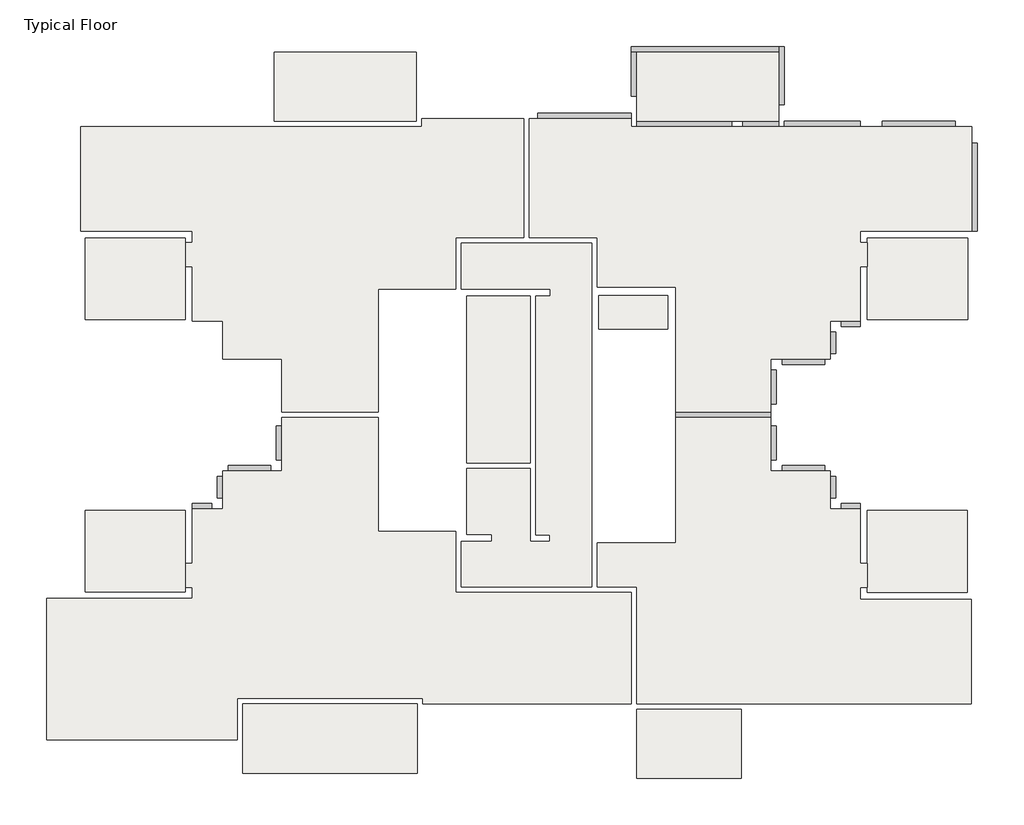
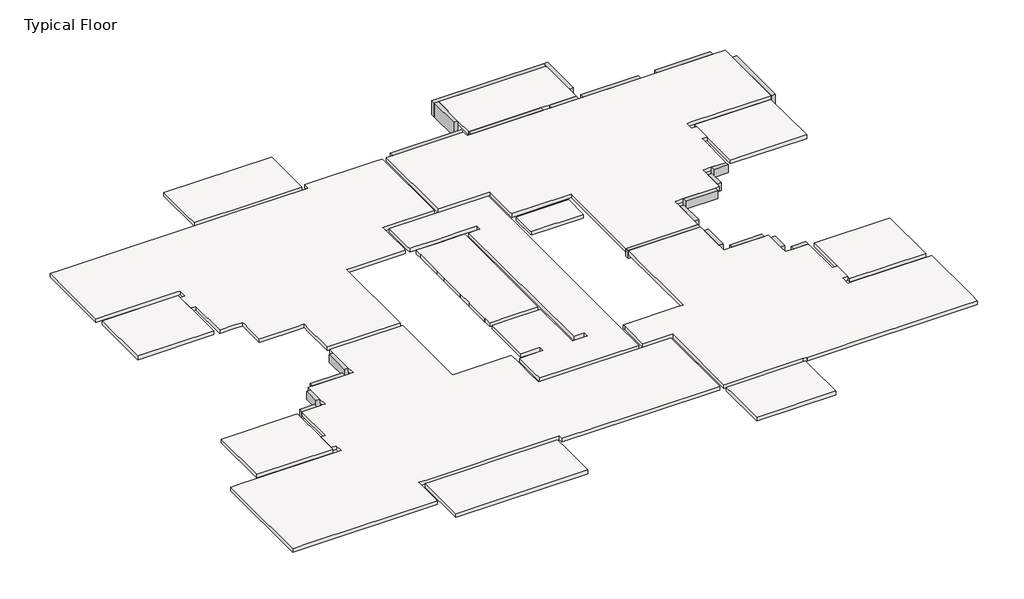
# One storey: 22 beams, 15 slabs.
"""IFC4 building model written with IfcOpenShell, lengths in millimetres."""

import ifcopenshell
import ifcopenshell.guid

model = None  # the IFC model being written
_history = None  # IfcOwnerHistory: only IFC2X3 demands one
_inside = {}  # id of a spatial element -> (the spatial element, [elements in it])
_under = {}  # id of a project, library or spatial element -> (it, [spatial elements below it])
_declared = {}  # id of a project -> (the project, [libraries it declares])
_typed = {}  # id of a type object -> (the type object, [elements of that type])
_made_of = {}  # id of a material, layer set ... -> (it, [elements and type objects made of it])


def new_model(schema):
    """Start an empty IFC model of exactly this schema.

    Asked for "IFC4X3", IfcOpenShell would pick the latest addendum, in which some entities
    have other attributes; the version numbers below select the first issue.
    IFC2X3 requires an IfcOwnerHistory on every rooted entity: one is made here for all.
    """
    global model, _history
    if schema == "IFC4X3":
        model = ifcopenshell.file(schema_version=(4, 3, 0, 0))
    else:
        model = ifcopenshell.file(schema=schema)
    _inside.clear()
    _under.clear()
    _declared.clear()
    _typed.clear()
    _made_of.clear()
    _history = None
    if model.schema == "IFC2X3":
        org = make("IfcOrganization", Name="unknown")
        user = make(
            "IfcPersonAndOrganization",
            ThePerson=make("IfcPerson", FamilyName="unknown"),
            TheOrganization=org,
        )
        app = make(
            "IfcApplication",
            ApplicationDeveloper=org,
            Version="unknown",
            ApplicationFullName="unknown",
            ApplicationIdentifier="unknown",
        )
        _history = make(
            "IfcOwnerHistory",
            OwningUser=user,
            OwningApplication=app,
            ChangeAction="ADDED",
            CreationDate=0,
        )
    return model


def make(cls, **values):
    """One entity of the class cls with the attributes given. An attribute that is None is left unset."""
    return model.create_entity(
        cls, **{name: value for name, value in values.items() if value is not None}
    )


def rooted(cls, **values):
    """An entity with a GlobalId (a new one), such as an element, a storey or a relation."""
    return make(cls, GlobalId=ifcopenshell.guid.new(), OwnerHistory=_history, **values)


def si_unit(unit_type, name, prefix=None):
    """IfcSIUnit, for example si_unit("LENGTHUNIT", "METRE", prefix="MILLI")."""
    return make("IfcSIUnit", UnitType=unit_type, Prefix=prefix, Name=name)


def assignment(units):
    """IfcUnitAssignment: the units of a project."""
    return None if units is None else make("IfcUnitAssignment", Units=units)


def point(xyz):
    """IfcCartesianPoint."""
    return None if xyz is None else make("IfcCartesianPoint", Coordinates=xyz)


def direction(xyz):
    """IfcDirection."""
    return None if xyz is None else make("IfcDirection", DirectionRatios=xyz)


def frame(location, z_axis=None, x_axis=None):
    """IfcAxis2Placement3D, a coordinate frame: its origin and axes. An axis left out is left unset."""
    return make(
        "IfcAxis2Placement3D",
        Location=point(location),
        Axis=direction(z_axis),
        RefDirection=direction(x_axis),
    )


def origin():
    """The frame at (0, 0, 0) with its axes left unset."""
    return frame((0.0, 0.0, 0.0))


def place(relative_to, where):
    """IfcLocalPlacement: puts the frame where relative to a parent placement (None: the world)."""
    return make(
        "IfcLocalPlacement", PlacementRelTo=relative_to, RelativePlacement=where
    )


def context(
    kind, dimensions, precision=None, world=None, true_north=None, identifier=None
):
    """IfcGeometricRepresentationContext, for example the 3D "Model" context."""
    return make(
        "IfcGeometricRepresentationContext",
        ContextIdentifier=identifier,
        ContextType=kind,
        CoordinateSpaceDimension=dimensions,
        Precision=precision,
        WorldCoordinateSystem=world,
        TrueNorth=true_north,
    )


def project(units=None, contexts=None):
    """IfcProject with its units and contexts."""
    return rooted(
        "IfcProject",
        Name="project",
        RepresentationContexts=contexts,
        UnitsInContext=assignment(units),
    )


def spatial(cls, under=None, at=None, **own):
    """A site, building, storey or space (cls), placed at a placement, below another one or the project."""
    s = rooted(cls, ObjectPlacement=at, **own)
    if under is not None:
        _under.setdefault(under.id(), (under, []))[1].append(s)
    return s


def polyline(points):
    """IfcPolyline through the points."""
    return make("IfcPolyline", Points=[point(p) for p in points])


def outline(outer, holes=None, kind="AREA"):
    """IfcArbitraryClosedProfileDef: a profile drawn as a closed curve; with holes, ...WithVoids."""
    if holes is None:
        return make("IfcArbitraryClosedProfileDef", ProfileType=kind, OuterCurve=outer)
    return make(
        "IfcArbitraryProfileDefWithVoids",
        ProfileType=kind,
        OuterCurve=outer,
        InnerCurves=holes,
    )


def extrude(swept, where, along, depth):
    """IfcExtrudedAreaSolid: the profile swept, set in the frame where, extruded along a direction by depth."""
    return make(
        "IfcExtrudedAreaSolid",
        SweptArea=swept,
        Position=where,
        ExtrudedDirection=direction(along),
        Depth=depth,
    )


def faces_of(points, faces, orient=None, outer=None):
    """IfcFace entities. A face is a list of loops; a loop is a list of indices into points, from 0.

    orient and outer hold one flag for each loop. By default every Orientation is true, the
    first loop of a face is its IfcFaceOuterBound and the others are IfcFaceBound.
    """
    made = []
    for i, loops in enumerate(faces):
        bounds = []
        for j, loop in enumerate(loops):
            is_outer = j == 0 if outer is None else outer[i][j]
            bounds.append(
                make(
                    "IfcFaceOuterBound" if is_outer else "IfcFaceBound",
                    Bound=make("IfcPolyLoop", Polygon=[points[k] for k in loop]),
                    Orientation=True if orient is None else orient[i][j],
                )
            )
        made.append(make("IfcFace", Bounds=bounds))
    return made


def faceted_brep(points, faces, orient=None, outer=None, voids=None):
    """IfcFacetedBrep: a solid bounded by flat faces; with voids (closed shells), ...WithVoids."""
    shared = [point(p) for p in points]
    hull = make("IfcClosedShell", CfsFaces=faces_of(shared, faces, orient, outer))
    if voids is None:
        return make("IfcFacetedBrep", Outer=hull)
    return make(
        "IfcFacetedBrepWithVoids",
        Outer=hull,
        Voids=[
            make(cls, CfsFaces=faces_of(shared, fs, o, b)) for cls, fs, o, b in voids
        ],
    )


def shape(context_of_items, identifier, shape_type, items):
    """IfcShapeRepresentation: the items that make up one representation, for example the "Body"."""
    return make(
        "IfcShapeRepresentation",
        ContextOfItems=context_of_items,
        RepresentationIdentifier=identifier,
        RepresentationType=shape_type,
        Items=items,
    )


def made_of(thing, what):
    """Note that an element or type object is made of a material, layer set ...; save() writes the relation."""
    if what is not None:
        _made_of.setdefault(what.id(), (what, []))[1].append(thing)
    return thing


def element(
    cls,
    number,
    at=None,
    inside=None,
    cuts=None,
    type_object=None,
    material=None,
    context=None,
    identifier="Body",
    shape_type=None,
    held_by="IfcProductDefinitionShape",
    body=None,
    shapes=None,
    **own,
):
    """One element of the class cls, such as IfcWall. Its Tag is "e" and its number.

    at: its placement. inside: the storey or other place that contains it. cuts: it is an
    opening in that element (IfcRelVoidsElement). A single representation is given by context,
    identifier, shape_type and body (its items); several are given by shapes. held_by: the class
    of the entity that holds the representations. save() writes the other relations.
    """
    e = rooted(cls, Tag="e%d" % number, ObjectPlacement=at, **own)
    if body is not None:
        shapes = [shape(context, identifier, shape_type, body)]
    if shapes is not None:
        e.Representation = make(held_by, Representations=shapes)
    if inside is not None:
        _inside.setdefault(inside.id(), (inside, []))[1].append(e)
    if cuts is not None:
        rooted(
            "IfcRelVoidsElement", RelatingBuildingElement=cuts, RelatedOpeningElement=e
        )
    if type_object is not None:
        _typed.setdefault(type_object.id(), (type_object, []))[1].append(e)
    return made_of(e, material)


def aggregate(whole, parts):
    """IfcRelAggregates: a whole, such as a stair, and the parts it consists of."""
    return rooted("IfcRelAggregates", RelatingObject=whole, RelatedObjects=parts)


def save(model, path):
    """Write the relations noted so far, then the file.

    IfcRelAggregates (storeys below a building ...), IfcRelContainedInSpatialStructure (elements
    in a storey), IfcRelDefinesByType, IfcRelAssociatesMaterial and IfcRelDeclares: one each for
    every whole, place, type object, material and project.
    """
    for whole, parts in _under.values():
        aggregate(whole, parts)
    for where, things in _inside.values():
        rooted(
            "IfcRelContainedInSpatialStructure",
            RelatedElements=things,
            RelatingStructure=where,
        )
    for kind, things in _typed.values():
        rooted("IfcRelDefinesByType", RelatedObjects=things, RelatingType=kind)
    for what, things in _made_of.values():
        rooted("IfcRelAssociatesMaterial", RelatedObjects=things, RelatingMaterial=what)
    for by, libraries in _declared.values():
        rooted("IfcRelDeclares", RelatingContext=by, RelatedDefinitions=libraries)
    model.write(path)


model = new_model("IFC4")

# Units and contexts
model_context = context("Model", 3, world=origin())
ifc_project = project(units=[si_unit("LENGTHUNIT", "METRE", prefix="MILLI")], contexts=[model_context])

# Site, building, storey
site = spatial("IfcSite", under=ifc_project)
building = spatial("IfcBuilding", under=site)
storey = spatial("IfcBuildingStorey", under=building, Name="Typical Floor", Elevation=3200.0)

# Beams
placement = place(None, origin())
element("IfcBeam", 1, ObjectType="Concrete Rectengular Beam : 20/40", at=placement, inside=storey, context=model_context, shape_type="Brep", body=[
    faceted_brep([(12187.8813243, 1505.2784849, 3200.0), (12187.8813243, 1705.2784849, 3200.0), (11489.3591568, 1705.2784849, 3200.0), (11489.3591568, 1505.2784849, 3200.0), (12187.8813243, 1705.2784849, 3020.0), (12187.8813243, 1705.2784849, 2800.0), (11489.3591568, 1705.2784849, 2800.0), (12187.8813243, 1505.2784849, 2800.0), (11489.3591568, 1505.2784849, 2800.0)], [[[0, 1, 2, 3]], [[1, 4, 5, 6, 2]], [[5, 7, 8, 6]], [[7, 0, 3, 8]], [[1, 0, 7, 5, 4]], [[3, 2, 6, 8]]]),
])
element("IfcBeam", 2, ObjectType="Concrete Rectengular Beam : 20/40", at=placement, inside=storey, context=model_context, shape_type="SweptSolid", body=[
    extrude(outline(polyline([(11289.3591568, 525.2784849), (11089.3591568, 525.2784849), (11089.3591568, 1305.2784849), (11289.3591568, 1305.2784849), (11289.3591568, 525.2784849)])), frame((0.0, 0.0, 2800.0), z_axis=(0.0, 0.0, 1.0), x_axis=(1.0, 0.0, 0.0)), (0.0, 0.0, 1.0), 400.0),
])
element("IfcBeam", 3, ObjectType="Concrete Rectengular Beam : 20/40", at=placement, inside=storey, context=model_context, shape_type="SweptSolid", body=[
    extrude(outline(polyline([(9356.052096, 125.2784849), (9356.052096, 325.2784849), (10889.3591568, 325.2784849), (10889.3591568, 125.2784849), (9356.052096, 125.2784849)])), frame((0.0, 0.0, 2800.0), z_axis=(0.0, 0.0, 1.0), x_axis=(1.0, 0.0, 0.0)), (0.0, 0.0, 1.0), 400.0),
])
element("IfcBeam", 4, ObjectType="Concrete Rectengular Beam : 20/40", at=placement, inside=storey, context=model_context, shape_type="Brep", body=[
    faceted_brep([(8956.052096, -1293.9530422, 3200.0), (9156.052096, -1293.9530422, 3200.0), (9156.052096, -74.7215151, 3200.0), (8956.052096, -74.7215151, 3200.0), (9156.052096, -1293.9530422, 2800.0), (9156.052096, -74.7215151, 2800.0), (8956.052096, -1293.9530422, 2800.0), (8956.052096, -74.7215151, 2800.0), (8956.052096, -1293.9530422, 3020.0)], [[[0, 1, 2, 3]], [[1, 4, 5, 2]], [[4, 6, 7, 5]], [[6, 8, 0, 3, 7]], [[1, 0, 8, 6, 4]], [[3, 2, 5, 7]]]),
])
element("IfcBeam", 5, ObjectType="Concrete Rectengular Beam : 20/40", at=placement, inside=storey, context=model_context, shape_type="Brep", body=[
    faceted_brep([(8956.052096, -1793.9530422, 3200.0), (8956.052096, -1593.9530422, 3200.0), (5525.8815794, -1593.9530422, 3200.0), (5525.8815794, -1793.9530422, 3200.0), (8956.052096, -1793.9530422, 2800.0), (8956.052096, -1793.9530422, 3020.0), (5525.8815794, -1793.9530422, 3020.0), (5525.8815794, -1793.9530422, 2800.0), (8956.052096, -1593.9530422, 2800.0), (5525.8815794, -1593.9530422, 2800.0), (8956.052096, -1593.9530422, 3020.0), (5525.8815794, -1593.9530422, 3020.0)], [[[0, 1, 2, 3]], [[4, 5, 0, 3, 6, 7]], [[8, 4, 7, 9]], [[1, 10, 8, 9, 11, 2]], [[1, 0, 5, 4, 8, 10]], [[3, 2, 11, 9, 7, 6]]]),
])
element("IfcBeam", 6, ObjectType="Concrete Rectengular Beam : 20/40", at=placement, inside=storey, context=model_context, shape_type="Brep", body=[
    faceted_brep([(-11929.8186713, -4893.1845693, 3200.0), (-11929.8186713, -5093.1845693, 3200.0), (-11231.2965038, -5093.1845693, 3200.0), (-11231.2965038, -4893.1845693, 3200.0), (-11929.8186713, -5093.1845693, 3020.0), (-11929.8186713, -5093.1845693, 2800.0), (-11231.2965038, -5093.1845693, 2800.0), (-11929.8186713, -4893.1845693, 2800.0), (-11231.2965038, -4893.1845693, 2800.0)], [[[0, 1, 2, 3]], [[1, 4, 5, 6, 2]], [[5, 7, 8, 6]], [[7, 0, 3, 8]], [[1, 0, 7, 5, 4]], [[3, 2, 6, 8]]]),
])
element("IfcBeam", 7, ObjectType="Concrete Rectengular Beam : 20/40", at=placement, inside=storey, context=model_context, shape_type="SweptSolid", body=[
    extrude(outline(polyline([(-11031.2965038, -3913.1845693), (-10831.2965038, -3913.1845693), (-10831.2965038, -4693.1845693), (-11031.2965038, -4693.1845693), (-11031.2965038, -3913.1845693)])), frame((0.0, 0.0, 2800.0), z_axis=(0.0, 0.0, 1.0), x_axis=(1.0, 0.0, 0.0)), (0.0, 0.0, 1.0), 400.0),
])
element("IfcBeam", 8, ObjectType="Concrete Rectengular Beam : 20/40", at=placement, inside=storey, context=model_context, shape_type="SweptSolid", body=[
    extrude(outline(polyline([(-9097.9894431, -3513.1845693), (-9097.9894431, -3713.1845693), (-10631.2965038, -3713.1845693), (-10631.2965038, -3513.1845693), (-9097.9894431, -3513.1845693)])), frame((0.0, 0.0, 2800.0), z_axis=(0.0, 0.0, 1.0), x_axis=(1.0, 0.0, 0.0)), (0.0, 0.0, 1.0), 400.0),
])
element("IfcBeam", 9, ObjectType="Concrete Rectengular Beam : 20/40", at=placement, inside=storey, context=model_context, shape_type="Brep", body=[
    faceted_brep([(-8697.9894431, -2093.9530422, 3200.0), (-8897.9894431, -2093.9530422, 3200.0), (-8897.9894431, -3313.1845693, 3200.0), (-8697.9894431, -3313.1845693, 3200.0), (-8897.9894431, -2093.9530422, 2800.0), (-8897.9894431, -3313.1845693, 2800.0), (-8697.9894431, -2093.9530422, 2800.0), (-8697.9894431, -3313.1845693, 2800.0), (-8697.9894431, -2093.9530422, 3020.0)], [[[0, 1, 2, 3]], [[1, 4, 5, 2]], [[4, 6, 7, 5]], [[6, 8, 0, 3, 7]], [[1, 0, 8, 6, 4]], [[3, 2, 5, 7]]]),
])
element("IfcBeam", 10, ObjectType="Concrete Rectengular Beam : 20/40", at=placement, inside=storey, context=model_context, shape_type="Brep", body=[
    faceted_brep([(12187.8813243, -5093.1845693, 3200.0), (12187.8813243, -4893.1845693, 3200.0), (11489.3591568, -4893.1845693, 3200.0), (11489.3591568, -5093.1845693, 3200.0), (12187.8813243, -5093.1845693, 2800.0), (12187.8813243, -5093.1845693, 3020.0), (11489.3591568, -5093.1845693, 2800.0), (12187.8813243, -4893.1845693, 2800.0), (11489.3591568, -4893.1845693, 2800.0)], [[[0, 1, 2, 3]], [[4, 5, 0, 3, 6]], [[7, 4, 6, 8]], [[1, 7, 8, 2]], [[1, 0, 5, 4, 7]], [[3, 2, 8, 6]]]),
])
element("IfcBeam", 11, ObjectType="Concrete Rectengular Beam : 20/40", at=placement, inside=storey, context=model_context, shape_type="SweptSolid", body=[
    extrude(outline(polyline([(11289.3591568, -4693.1845693), (11089.3591568, -4693.1845693), (11089.3591568, -3913.1845693), (11289.3591568, -3913.1845693), (11289.3591568, -4693.1845693)])), frame((0.0, 0.0, 2800.0), z_axis=(0.0, 0.0, 1.0), x_axis=(1.0, 0.0, 0.0)), (0.0, 0.0, 1.0), 400.0),
])
element("IfcBeam", 12, ObjectType="Concrete Rectengular Beam : 20/40", at=placement, inside=storey, context=model_context, shape_type="SweptSolid", body=[
    extrude(outline(polyline([(10889.3591568, -3513.1845693), (10889.3591568, -3713.1845693), (9356.052096, -3713.1845693), (9356.052096, -3513.1845693), (10889.3591568, -3513.1845693)])), frame((0.0, 0.0, 2800.0), z_axis=(0.0, 0.0, 1.0), x_axis=(1.0, 0.0, 0.0)), (0.0, 0.0, 1.0), 400.0),
])
element("IfcBeam", 13, ObjectType="Concrete Rectengular Beam : 20/40", at=placement, inside=storey, context=model_context, shape_type="Brep", body=[
    faceted_brep([(9156.052096, -2093.9530422, 3200.0), (8956.052096, -2093.9530422, 3200.0), (8956.052096, -3313.1845693, 3200.0), (9156.052096, -3313.1845693, 3200.0), (9156.052096, -2093.9530422, 2800.0), (9156.052096, -3313.1845693, 2800.0), (8956.052096, -2093.9530422, 2800.0), (8956.052096, -3313.1845693, 2800.0), (8956.052096, -2093.9530422, 3020.0)], [[[0, 1, 2, 3]], [[4, 0, 3, 5]], [[6, 4, 5, 7]], [[1, 8, 6, 7, 2]], [[1, 0, 4, 6, 8]], [[3, 2, 7, 5]]]),
])
element("IfcBeam", 14, ObjectType="Concrete Rectengular Beam : 20/50", at=placement, inside=storey, context=model_context, shape_type="Brep", body=[
    faceted_brep([(4107.8539459, 8914.1448811, 3200.0), (4107.8539459, 8714.1448811, 3200.0), (7543.9303787, 8714.1448811, 3200.0), (7543.9303787, 8914.1448811, 3200.0), (4107.8539459, 8914.1448811, 2700.0), (4107.8539459, 8914.1448811, 3020.0), (7543.9303787, 8914.1448811, 2700.0), (4107.8539459, 8714.1448811, 2700.0), (7543.9303787, 8714.1448811, 2700.0), (4107.8539459, 8714.1448811, 3020.0), (7543.9303787, 8714.1448811, 3020.0)], [[[0, 1, 2, 3]], [[4, 5, 0, 3, 6]], [[7, 4, 6, 8]], [[2, 1, 9, 7, 8, 10]], [[1, 0, 5, 4, 7, 9]], [[3, 2, 10, 8, 6]]]),
])
element("IfcBeam", 15, ObjectType="Concrete Rectengular Beam : 20/50", at=placement, inside=storey, context=model_context, shape_type="Brep", body=[
    faceted_brep([(7943.9303787, 8914.1448811, 3200.0), (7943.9303787, 8714.1448811, 3200.0), (9233.1802646, 8714.1448811, 3200.0), (9233.1802646, 8914.1448811, 3200.0), (7943.9303787, 8914.1448811, 2700.0), (9233.1802646, 8914.1448811, 3020.0), (9233.1802646, 8914.1448811, 2700.0), (7943.9303787, 8714.1448811, 2700.0), (9233.1802646, 8714.1448811, 2700.0), (7943.9303787, 8714.1448811, 3020.0), (9233.1802646, 8714.1448811, 3020.0)], [[[0, 1, 2, 3]], [[4, 0, 3, 5, 6]], [[7, 4, 6, 8]], [[2, 1, 9, 7, 8, 10]], [[1, 0, 4, 7, 9]], [[3, 2, 10, 8, 6, 5]]]),
])
element("IfcBeam", 16, ObjectType="Concrete Rectengular Beam : 20/50", at=placement, inside=storey, context=model_context, shape_type="Brep", body=[
    faceted_brep([(9433.1802646, 8914.1448811, 3200.0), (9433.1802646, 8714.1448811, 3200.0), (12172.2581695, 8714.1448811, 3200.0), (12172.2581695, 8914.1448811, 3200.0), (9433.1802646, 8914.1448811, 2700.0), (12172.2581695, 8914.1448811, 2700.0), (9433.1802646, 8714.1448811, 2700.0), (12172.2581695, 8714.1448811, 2700.0), (9433.1802646, 8714.1448811, 3020.0), (12172.2581695, 8714.1448811, 3020.0)], [[[0, 1, 2, 3]], [[4, 0, 3, 5]], [[6, 4, 5, 7]], [[2, 1, 8, 6, 7, 9]], [[1, 0, 4, 6, 8]], [[3, 2, 9, 7, 5]]]),
])
element("IfcBeam", 17, ObjectType="Concrete Rectengular Beam : 20/50", at=placement, inside=storey, context=model_context, shape_type="Brep", body=[
    faceted_brep([(12972.2581695, 8914.1448811, 3200.0), (12972.2581695, 8714.1448811, 3200.0), (15617.6251666, 8714.1448811, 3200.0), (15617.6251666, 8914.1448811, 3200.0), (12972.2581695, 8914.1448811, 2700.0), (15617.6251666, 8914.1448811, 2700.0), (12972.2581695, 8714.1448811, 2700.0), (15617.6251666, 8714.1448811, 2700.0), (12972.2581695, 8714.1448811, 3020.0), (15617.6251666, 8714.1448811, 3020.0)], [[[0, 1, 2, 3]], [[4, 0, 3, 5]], [[6, 4, 5, 7]], [[2, 1, 8, 6, 7, 9]], [[1, 0, 4, 6, 8]], [[3, 2, 9, 7, 5]]]),
])
element("IfcBeam", 18, ObjectType="Concrete Rectengular Beam : 20/50", at=placement, inside=storey, context=model_context, shape_type="Brep", body=[
    faceted_brep([(16410.4478267, 8125.9123109, 3200.0), (16210.4478267, 8125.9123109, 3200.0), (16210.4478267, 4939.6791417, 3200.0), (16410.4478267, 4939.6791417, 3200.0), (16410.4478267, 8125.9123109, 2700.0), (16410.4478267, 4939.6791417, 2700.0), (16210.4478267, 8125.9123109, 2700.0), (16210.4478267, 4939.6791417, 2700.0), (16210.4478267, 4939.6791417, 3020.0)], [[[0, 1, 2, 3]], [[4, 0, 3, 5]], [[6, 4, 5, 7]], [[1, 6, 7, 8, 2]], [[1, 0, 4, 6]], [[3, 2, 8, 7, 5]]]),
])
element("IfcBeam", 19, ObjectType="Concrete Rectengular Beam : 20/50", at=placement, inside=storey, context=model_context, shape_type="Brep", body=[
    faceted_brep([(3907.8539459, 9014.1448811, 3200.0), (3907.8539459, 9214.1448811, 3200.0), (529.0313265, 9214.1448811, 3200.0), (529.0313265, 9014.1448811, 3200.0), (3907.8539459, 9214.1448811, 2700.0), (529.0313265, 9214.1448811, 2700.0), (3907.8539459, 9014.1448811, 2700.0), (529.0313265, 9014.1448811, 2700.0), (3907.8539459, 9014.1448811, 3020.0)], [[[0, 1, 2, 3]], [[1, 4, 5, 2]], [[4, 6, 7, 5]], [[6, 8, 0, 3, 7]], [[1, 0, 8, 6, 4]], [[3, 2, 5, 7]]]),
])
element("IfcBeam", 20, ObjectType="Concrete Rectengular Beam : 20/70", at=placement, inside=storey, context=model_context, shape_type="Brep", body=[
    faceted_brep([(9433.1802646, 11614.1448811, 3200.0), (9233.1802646, 11614.1448811, 3200.0), (9233.1802646, 11414.1448811, 3200.0), (9233.1802646, 9514.1448811, 3200.0), (9433.1802646, 9514.1448811, 3200.0), (9233.1802646, 11614.1448811, 2500.0), (9233.1802646, 11414.1448811, 2500.0), (9233.1802646, 9514.1448811, 2500.0), (9433.1802646, 11614.1448811, 2500.0), (9433.1802646, 9514.1448811, 2500.0)], [[[0, 1, 2, 3, 4]], [[1, 5, 6, 7, 3, 2]], [[5, 8, 9, 7, 6]], [[8, 0, 4, 9]], [[4, 3, 7, 9]], [[1, 0, 8, 5]]]),
])
element("IfcBeam", 21, ObjectType="Concrete Rectengular Beam : 20/70", at=placement, inside=storey, context=model_context, shape_type="Brep", body=[
    faceted_brep([(3907.8539459, 11614.1448811, 3200.0), (3907.8539459, 11414.1448811, 3200.0), (4107.8539459, 11414.1448811, 3200.0), (9233.1802646, 11414.1448811, 3200.0), (9233.1802646, 11614.1448811, 3200.0), (3907.8539459, 11414.1448811, 2500.0), (4107.8539459, 11414.1448811, 2500.0), (9233.1802646, 11414.1448811, 2500.0), (9233.1802646, 11414.1448811, 3020.0), (3907.8539459, 11614.1448811, 2500.0), (9233.1802646, 11614.1448811, 2500.0)], [[[0, 1, 2, 3, 4]], [[1, 5, 6, 7, 8, 3, 2]], [[5, 9, 10, 7, 6]], [[9, 0, 4, 10]], [[4, 3, 8, 7, 10]], [[1, 0, 9, 5]]]),
])
element("IfcBeam", 22, ObjectType="Concrete Rectengular Beam : 20/70", at=placement, inside=storey, context=model_context, shape_type="Brep", body=[
    faceted_brep([(3907.8539459, 9814.1448811, 3200.0), (4107.8539459, 9814.1448811, 3200.0), (4107.8539459, 11414.1448811, 3200.0), (3907.8539459, 11414.1448811, 3200.0), (4107.8539459, 9814.1448811, 2500.0), (4107.8539459, 11414.1448811, 2500.0), (4107.8539459, 11414.1448811, 3020.0), (3907.8539459, 9814.1448811, 2500.0), (3907.8539459, 11414.1448811, 2500.0)], [[[0, 1, 2, 3]], [[1, 4, 5, 6, 2]], [[4, 7, 8, 5]], [[7, 0, 3, 8]], [[1, 0, 7, 4]], [[3, 2, 6, 5, 8]]]),
])

# Slabs
element("IfcSlab", 23, ObjectType="18", at=placement, inside=storey, context=model_context, shape_type="Brep", body=[
    faceted_brep([(-12179.8186713, 4689.6791417, 3020.0), (-12179.8186713, 4539.6791417, 3020.0), (-12179.8186713, 3668.3687969, 3020.0), (-12179.8186713, 1755.2784849, 3020.0), (-15802.3851738, 1755.2784849, 3020.0), (-15802.3851738, 4689.6791417, 3020.0), (-12179.8186713, 4689.6791417, 3200.0), (-15802.3851738, 4689.6791417, 3200.0), (-15802.3851738, 1755.2784849, 3200.0), (-12179.8186713, 1755.2784849, 3200.0), (-12179.8186713, 3668.3687969, 3200.0), (-12179.8186713, 4539.6791417, 3200.0)], [[[0, 1, 2, 3, 4, 5]], [[6, 7, 8, 9, 10, 11]], [[3, 2, 1, 0, 6, 11, 10, 9]], [[4, 3, 9, 8]], [[5, 4, 8, 7]], [[0, 5, 7, 6]]]),
])
element("IfcSlab", 24, ObjectType="18", at=placement, inside=storey, context=model_context, shape_type="Brep", body=[
    faceted_brep([(-15952.3851738, 4939.6791417, 3020.0), (-15952.3851738, 8714.1448811, 3020.0), (-15359.5625137, 8714.1448811, 3020.0), (-11484.1955166, 8714.1448811, 3020.0), (-10684.1955166, 8714.1448811, 3020.0), (-9175.1176117, 8714.1448811, 3020.0), (-8975.1176117, 8714.1448811, 3020.0), (-7685.8677257, 8714.1448811, 3020.0), (-7285.8677257, 8714.1448811, 3020.0), (-3849.7912929, 8714.1448811, 3020.0), (-3649.7912929, 8714.1448811, 3020.0), (-3649.7912929, 9014.1448811, 3020.0), (29.0313265, 9014.1448811, 3020.0), (29.0313265, 4709.9784533, 3020.0), (-2215.274667, 4709.9784533, 3020.0), (-2415.274667, 4709.9784533, 3020.0), (-2415.274667, 4069.9784533, 3020.0), (-2415.274667, 3043.8247791, 3020.0), (-2415.274667, 2858.8247791, 3020.0), (-4927.8189264, 2858.8247791, 3020.0), (-5227.8189264, 2858.8247791, 3020.0), (-5227.8189264, -1593.9530422, 3020.0), (-8697.9894431, -1593.9530422, 3020.0), (-8697.9894431, -1293.9530422, 3020.0), (-8697.9894431, -74.7215151, 3020.0), (-8697.9894431, 325.2784849, 3020.0), (-9097.9894431, 325.2784849, 3020.0), (-10631.2965038, 325.2784849, 3020.0), (-10831.2965038, 325.2784849, 3020.0), (-10831.2965038, 525.2784849, 3020.0), (-10831.2965038, 1285.2784849, 3020.0), (-10831.2965038, 1505.2784849, 3020.0), (-10831.2965038, 1705.2784849, 3020.0), (-11231.2965038, 1705.2784849, 3020.0), (-11929.8186713, 1705.2784849, 3020.0), (-11929.8186713, 3668.3687969, 3020.0), (-12179.8186713, 3668.3687969, 3020.0), (-12179.8186713, 4539.6791417, 3020.0), (-11929.8186713, 4539.6791417, 3020.0), (-11929.8186713, 4939.6791417, 3020.0), (-12179.8186713, 4939.6791417, 3020.0), (-15952.3851738, 8714.1448811, 3200.0), (-15952.3851738, 8125.9123109, 3200.0), (-15952.3851738, 4939.6791417, 3200.0), (-12179.8186713, 4939.6791417, 3200.0), (-11929.8186713, 4939.6791417, 3200.0), (-11929.8186713, 4539.6791417, 3200.0), (-12179.8186713, 4539.6791417, 3200.0), (-12179.8186713, 3668.3687969, 3200.0), (-11929.8186713, 3668.3687969, 3200.0), (-11929.8186713, 1705.2784849, 3200.0), (-11231.2965038, 1705.2784849, 3200.0), (-10831.2965038, 1705.2784849, 3200.0), (-10831.2965038, 1505.2784849, 3200.0), (-10831.2965038, 1285.2784849, 3200.0), (-10831.2965038, 525.2784849, 3200.0), (-10831.2965038, 325.2784849, 3200.0), (-10631.2965038, 325.2784849, 3200.0), (-9097.9894431, 325.2784849, 3200.0), (-8697.9894431, 325.2784849, 3200.0), (-8697.9894431, -74.7215151, 3200.0), (-8697.9894431, -1293.9530422, 3200.0), (-8697.9894431, -1593.9530422, 3200.0), (-5227.8189264, -1593.9530422, 3200.0), (-5227.8189264, 2858.8247791, 3200.0), (-4927.8189264, 2858.8247791, 3200.0), (-2415.274667, 2858.8247791, 3200.0), (-2415.274667, 3043.8247791, 3200.0), (-2415.274667, 4069.9784533, 3200.0), (-2415.274667, 4709.9784533, 3200.0), (-2215.274667, 4709.9784533, 3200.0), (29.0313265, 4709.9784533, 3200.0), (29.0313265, 9014.1448811, 3200.0), (-270.9686735, 9014.1448811, 3200.0), (-3649.7912929, 9014.1448811, 3200.0), (-3649.7912929, 8714.1448811, 3200.0), (-3849.7912929, 8714.1448811, 3200.0), (-7285.8677257, 8714.1448811, 3200.0), (-7685.8677257, 8714.1448811, 3200.0), (-8975.1176117, 8714.1448811, 3200.0), (-9175.1176117, 8714.1448811, 3200.0), (-10684.1955166, 8714.1448811, 3200.0), (-11484.1955166, 8714.1448811, 3200.0), (-15359.5625137, 8714.1448811, 3200.0)], [[[0, 1, 2, 3, 4, 5, 6, 7, 8, 9, 10, 11, 12, 13, 14, 15, 16, 17, 18, 19, 20, 21, 22, 23, 24, 25, 26, 27, 28, 29, 30, 31, 32, 33, 34, 35, 36, 37, 38, 39, 40]], [[41, 42, 43, 44, 45, 46, 47, 48, 49, 50, 51, 52, 53, 54, 55, 56, 57, 58, 59, 60, 61, 62, 63, 64, 65, 66, 67, 68, 69, 70, 71, 72, 73, 74, 75, 76, 77, 78, 79, 80, 81, 82, 83]], [[1, 0, 43, 42, 41]], [[1, 41, 83, 82, 81, 80, 79, 78, 77, 76, 75, 10, 9, 8, 7, 6, 5, 4, 3, 2]], [[11, 10, 75, 74]], [[12, 11, 74, 73, 72]], [[13, 12, 72, 71]], [[13, 71, 70, 69, 15, 14]], [[15, 69, 68, 67, 66, 18, 17, 16]], [[18, 66, 65, 64, 20, 19]], [[21, 20, 64, 63]], [[22, 21, 63, 62]], [[22, 62, 61, 60, 59, 25, 24, 23]], [[25, 59, 58, 57, 56, 28, 27, 26]], [[28, 56, 55, 54, 53, 52, 32, 31, 30, 29]], [[32, 52, 51, 50, 34, 33]], [[35, 34, 50, 49]], [[36, 35, 49, 48]], [[37, 36, 48, 47]], [[38, 37, 47, 46]], [[39, 38, 46, 45]], [[39, 45, 44, 43, 0, 40]]]),
])
element("IfcSlab", 25, ObjectType="18", at=placement, inside=storey, context=model_context, shape_type="Brep", body=[
    faceted_brep([(-3849.7912929, 11414.1448811, 3020.0), (-3849.7912929, 8914.1448811, 3020.0), (-8975.1176117, 8914.1448811, 3020.0), (-8975.1176117, 11414.1448811, 3020.0), (-3849.7912929, 8914.1448811, 3200.0), (-3849.7912929, 9814.1448811, 3200.0), (-3849.7912929, 11414.1448811, 3200.0), (-8975.1176117, 11414.1448811, 3200.0), (-8975.1176117, 9514.1448811, 3200.0), (-8975.1176117, 8914.1448811, 3200.0), (-7685.8677257, 8914.1448811, 3200.0), (-7285.8677257, 8914.1448811, 3200.0)], [[[0, 1, 2, 3]], [[4, 5, 6, 7, 8, 9, 10, 11]], [[1, 0, 6, 5, 4]], [[2, 1, 4, 11, 10, 9]], [[3, 2, 9, 8, 7]], [[0, 3, 7, 6]]]),
])
element("IfcSlab", 26, ObjectType="18", at=placement, inside=storey, context=model_context, shape_type="Brep", body=[
    faceted_brep([(12437.8813243, 4689.6791417, 3020.0), (16060.4478267, 4689.6791417, 3020.0), (16060.4478267, 1755.2784849, 3020.0), (12437.8813243, 1755.2784849, 3020.0), (12437.8813243, 3668.3687969, 3020.0), (12437.8813243, 4539.6791417, 3020.0), (12437.8813243, 4689.6791417, 3200.0), (12437.8813243, 4539.6791417, 3200.0), (12437.8813243, 3668.3687969, 3200.0), (12437.8813243, 1755.2784849, 3200.0), (16060.4478267, 1755.2784849, 3200.0), (16060.4478267, 4689.6791417, 3200.0)], [[[0, 1, 2, 3, 4, 5]], [[6, 7, 8, 9, 10, 11]], [[0, 5, 4, 3, 9, 8, 7, 6]], [[3, 2, 10, 9]], [[2, 1, 11, 10]], [[1, 0, 6, 11]]]),
])
element("IfcSlab", 27, ObjectType="18", at=placement, inside=storey, context=model_context, shape_type="Brep", body=[
    faceted_brep([(16210.4478267, 8714.1448811, 3020.0), (16210.4478267, 4939.6791417, 3020.0), (12437.8813243, 4939.6791417, 3020.0), (12187.8813243, 4939.6791417, 3020.0), (12187.8813243, 4539.6791417, 3020.0), (12437.8813243, 4539.6791417, 3020.0), (12437.8813243, 3668.3687969, 3020.0), (12187.8813243, 3668.3687969, 3020.0), (12187.8813243, 1705.2784849, 3020.0), (11489.3591568, 1705.2784849, 3020.0), (11089.3591568, 1705.2784849, 3020.0), (11089.3591568, 1305.2784849, 3020.0), (11089.3591568, 525.2784849, 3020.0), (11089.3591568, 325.2784849, 3020.0), (10889.3591568, 325.2784849, 3020.0), (9356.052096, 325.2784849, 3020.0), (8956.052096, 325.2784849, 3020.0), (8956.052096, -74.7215151, 3020.0), (8956.052096, -1293.9530422, 3020.0), (8956.052096, -1593.9530422, 3020.0), (5525.8815794, -1593.9530422, 3020.0), (5525.8815794, 2916.2932633, 3020.0), (5225.8815794, 2916.2932633, 3020.0), (2684.725333, 2916.2932633, 3020.0), (2684.725333, 3056.2932633, 3020.0), (2684.725333, 4049.9784533, 3020.0), (2684.725333, 4509.9784533, 3020.0), (2684.725333, 4709.9784533, 3020.0), (229.0313265, 4709.9784533, 3020.0), (229.0313265, 9014.1448811, 3020.0), (3907.8539459, 9014.1448811, 3020.0), (3907.8539459, 8714.1448811, 3020.0), (4107.8539459, 8714.1448811, 3020.0), (7543.9303787, 8714.1448811, 3020.0), (7943.9303787, 8714.1448811, 3020.0), (9233.1802646, 8714.1448811, 3020.0), (9433.1802646, 8714.1448811, 3020.0), (12172.2581695, 8714.1448811, 3020.0), (12972.2581695, 8714.1448811, 3020.0), (15617.6251666, 8714.1448811, 3020.0), (16210.4478267, 4939.6791417, 3200.0), (16210.4478267, 8125.9123109, 3200.0), (16210.4478267, 8714.1448811, 3200.0), (15617.6251666, 8714.1448811, 3200.0), (12972.2581695, 8714.1448811, 3200.0), (12172.2581695, 8714.1448811, 3200.0), (9433.1802646, 8714.1448811, 3200.0), (9233.1802646, 8714.1448811, 3200.0), (7943.9303787, 8714.1448811, 3200.0), (7543.9303787, 8714.1448811, 3200.0), (4107.8539459, 8714.1448811, 3200.0), (3907.8539459, 8714.1448811, 3200.0), (3907.8539459, 9014.1448811, 3200.0), (529.0313265, 9014.1448811, 3200.0), (229.0313265, 9014.1448811, 3200.0), (229.0313265, 4709.9784533, 3200.0), (2684.725333, 4709.9784533, 3200.0), (2684.725333, 4509.9784533, 3200.0), (2684.725333, 4049.9784533, 3200.0), (2684.725333, 3056.2932633, 3200.0), (2684.725333, 2916.2932633, 3200.0), (5225.8815794, 2916.2932633, 3200.0), (5525.8815794, 2916.2932633, 3200.0), (5525.8815794, -1593.9530422, 3200.0), (8956.052096, -1593.9530422, 3200.0), (8956.052096, -1293.9530422, 3200.0), (8956.052096, -74.7215151, 3200.0), (8956.052096, 325.2784849, 3200.0), (9356.052096, 325.2784849, 3200.0), (10889.3591568, 325.2784849, 3200.0), (11089.3591568, 325.2784849, 3200.0), (11089.3591568, 525.2784849, 3200.0), (11089.3591568, 1305.2784849, 3200.0), (11089.3591568, 1705.2784849, 3200.0), (11489.3591568, 1705.2784849, 3200.0), (12187.8813243, 1705.2784849, 3200.0), (12187.8813243, 3668.3687969, 3200.0), (12437.8813243, 3668.3687969, 3200.0), (12437.8813243, 4539.6791417, 3200.0), (12187.8813243, 4539.6791417, 3200.0), (12187.8813243, 4939.6791417, 3200.0), (12437.8813243, 4939.6791417, 3200.0)], [[[0, 1, 2, 3, 4, 5, 6, 7, 8, 9, 10, 11, 12, 13, 14, 15, 16, 17, 18, 19, 20, 21, 22, 23, 24, 25, 26, 27, 28, 29, 30, 31, 32, 33, 34, 35, 36, 37, 38, 39]], [[40, 41, 42, 43, 44, 45, 46, 47, 48, 49, 50, 51, 52, 53, 54, 55, 56, 57, 58, 59, 60, 61, 62, 63, 64, 65, 66, 67, 68, 69, 70, 71, 72, 73, 74, 75, 76, 77, 78, 79, 80, 81]], [[1, 0, 42, 41, 40]], [[31, 51, 50, 49, 48, 47, 46, 45, 44, 43, 42, 0, 39, 38, 37, 36, 35, 34, 33, 32]], [[31, 30, 52, 51]], [[30, 29, 54, 53, 52]], [[29, 28, 55, 54]], [[28, 27, 56, 55]], [[23, 60, 59, 58, 57, 56, 27, 26, 25, 24]], [[21, 62, 61, 60, 23, 22]], [[21, 20, 63, 62]], [[20, 19, 64, 63]], [[16, 67, 66, 65, 64, 19, 18, 17]], [[13, 70, 69, 68, 67, 16, 15, 14]], [[10, 73, 72, 71, 70, 13, 12, 11]], [[8, 75, 74, 73, 10, 9]], [[8, 7, 76, 75]], [[7, 6, 77, 76]], [[6, 5, 78, 77]], [[5, 4, 79, 78]], [[4, 3, 80, 79]], [[80, 3, 2, 1, 40, 81]]]),
])
element("IfcSlab", 28, ObjectType="18", at=placement, inside=storey, context=model_context, shape_type="Brep", body=[
    faceted_brep([(4107.8539459, 8914.1448811, 3020.0), (4107.8539459, 11414.1448811, 3020.0), (9233.1802646, 11414.1448811, 3020.0), (9233.1802646, 8914.1448811, 3020.0), (4107.8539459, 11414.1448811, 3200.0), (4107.8539459, 9814.1448811, 3200.0), (4107.8539459, 8914.1448811, 3200.0), (7543.9303787, 8914.1448811, 3200.0), (7943.9303787, 8914.1448811, 3200.0), (9233.1802646, 8914.1448811, 3200.0), (9233.1802646, 9514.1448811, 3200.0), (9233.1802646, 11414.1448811, 3200.0)], [[[0, 1, 2, 3]], [[4, 5, 6, 7, 8, 9, 10, 11]], [[1, 0, 6, 5, 4]], [[0, 3, 9, 8, 7, 6]], [[3, 2, 11, 10, 9]], [[2, 1, 4, 11]]]),
])
element("IfcSlab", 29, ObjectType="18", at=placement, inside=storey, context=model_context, shape_type="Brep", body=[
    faceted_brep([(-12179.8186713, -8077.5852261, 3020.0), (-15802.3851738, -8077.5852261, 3020.0), (-15802.3851738, -5143.1845693, 3020.0), (-12179.8186713, -5143.1845693, 3020.0), (-12179.8186713, -7056.2748812, 3020.0), (-12179.8186713, -7927.5852261, 3020.0), (-12179.8186713, -8077.5852261, 3200.0), (-12179.8186713, -7927.5852261, 3200.0), (-12179.8186713, -7056.2748812, 3200.0), (-12179.8186713, -5143.1845693, 3200.0), (-15802.3851738, -5143.1845693, 3200.0), (-15802.3851738, -8077.5852261, 3200.0)], [[[0, 1, 2, 3, 4, 5]], [[6, 7, 8, 9, 10, 11]], [[0, 5, 4, 3, 9, 8, 7, 6]], [[3, 2, 10, 9]], [[2, 1, 11, 10]], [[1, 0, 6, 11]]]),
])
element("IfcSlab", 30, ObjectType="18", at=placement, inside=storey, context=model_context, shape_type="Brep", body=[
    faceted_brep([(16040.4478267, -8097.5852261, 3020.0), (12437.8813243, -8097.5852261, 3020.0), (12437.8813243, -7927.5852261, 3020.0), (12437.8813243, -7056.2748812, 3020.0), (12437.8813243, -5143.1845693, 3020.0), (16040.4478267, -5143.1845693, 3020.0), (12437.8813243, -8097.5852261, 3200.0), (16040.4478267, -8097.5852261, 3200.0), (16040.4478267, -5143.1845693, 3200.0), (12437.8813243, -5143.1845693, 3200.0), (12437.8813243, -7056.2748812, 3200.0), (12437.8813243, -7927.5852261, 3200.0)], [[[0, 1, 2, 3, 4, 5]], [[6, 7, 8, 9, 10, 11]], [[1, 6, 11, 10, 9, 4, 3, 2]], [[7, 0, 5, 8]], [[1, 0, 7, 6]], [[5, 4, 9, 8]]]),
])
element("IfcSlab", 31, ObjectType="18", at=placement, inside=storey, context=model_context, shape_type="Brep", body=[
    faceted_brep([(-12179.8186713, -7056.2748812, 3020.0), (-11929.8186713, -7056.2748812, 3020.0), (-11929.8186713, -5093.1845693, 3020.0), (-11231.2965038, -5093.1845693, 3020.0), (-10831.2965038, -5093.1845693, 3020.0), (-10831.2965038, -4693.1845693, 3020.0), (-10831.2965038, -3913.1845693, 3020.0), (-10831.2965038, -3713.1845693, 3020.0), (-10631.2965038, -3713.1845693, 3020.0), (-9097.9894431, -3713.1845693, 3020.0), (-8697.9894431, -3713.1845693, 3020.0), (-8697.9894431, -3313.1845693, 3020.0), (-8697.9894431, -2093.9530422, 3020.0), (-8697.9894431, -1793.9530422, 3020.0), (-5227.8189264, -1793.9530422, 3020.0), (-5227.8189264, -5901.1752209, 3020.0), (-4927.8189264, -5901.1752209, 3020.0), (-2424.4804119, -5901.1752209, 3020.0), (-2424.4804119, -6461.1752209, 3020.0), (-2424.4804119, -7466.1752209, 3020.0), (-2424.4804119, -7911.1752209, 3020.0), (-2424.4804119, -8111.1752209, 3020.0), (3907.8539459, -8111.1752209, 3020.0), (3907.8539459, -12124.2691374, 3020.0), (529.0313265, -12124.2691374, 3020.0), (-270.9686735, -12124.2691374, 3020.0), (-3619.0362853, -12124.2691374, 3020.0), (-3619.0362853, -11921.300832, 3020.0), (-3819.0362853, -11921.300832, 3020.0), (-7004.989514, -11921.300832, 3020.0), (-7404.989514, -11921.300832, 3020.0), (-9913.9547043, -11921.300832, 3020.0), (-10303.9547043, -11921.300832, 3020.0), (-10303.9547043, -12121.300832, 3020.0), (-10303.9547043, -13432.1139628, 3020.0), (-17194.74029, -13432.1139628, 3020.0), (-17194.74029, -8327.5852261, 3020.0), (-16589.4316206, -8327.5852261, 3020.0), (-16152.3851738, -8327.5852261, 3020.0), (-12179.8186713, -8327.5852261, 3020.0), (-11929.8186713, -8327.5852261, 3020.0), (-11929.8186713, -7927.5852261, 3020.0), (-12179.8186713, -7927.5852261, 3020.0), (-11929.8186713, -7056.2748812, 3200.0), (-12179.8186713, -7056.2748812, 3200.0), (-12179.8186713, -7927.5852261, 3200.0), (-11929.8186713, -7927.5852261, 3200.0), (-11929.8186713, -8327.5852261, 3200.0), (-12179.8186713, -8327.5852261, 3200.0), (-16152.3851738, -8327.5852261, 3200.0), (-16589.4316206, -8327.5852261, 3200.0), (-17194.74029, -8327.5852261, 3200.0), (-17194.74029, -8893.4441313, 3200.0), (-17194.74029, -9493.6732518, 3200.0), (-17194.74029, -10293.6732518, 3200.0), (-17194.74029, -12822.7787814, 3200.0), (-17194.74029, -13432.1139628, 3200.0), (-16594.74029, -13432.1139628, 3200.0), (-13698.304807, -13432.1139628, 3200.0), (-12898.304807, -13432.1139628, 3200.0), (-10303.9547043, -13432.1139628, 3200.0), (-10303.9547043, -12121.300832, 3200.0), (-10303.9547043, -11921.300832, 3200.0), (-9913.9547043, -11921.300832, 3200.0), (-7404.989514, -11921.300832, 3200.0), (-7004.989514, -11921.300832, 3200.0), (-3819.0362853, -11921.300832, 3200.0), (-3619.0362853, -11921.300832, 3200.0), (-3619.0362853, -12124.2691374, 3200.0), (-270.9686735, -12124.2691374, 3200.0), (529.0313265, -12124.2691374, 3200.0), (3907.8539459, -12124.2691374, 3200.0), (3907.8539459, -8111.1752209, 3200.0), (-2424.4804119, -8111.1752209, 3200.0), (-2424.4804119, -7911.1752209, 3200.0), (-2424.4804119, -7466.1752209, 3200.0), (-2424.4804119, -6461.1752209, 3200.0), (-2424.4804119, -5901.1752209, 3200.0), (-4927.8189264, -5901.1752209, 3200.0), (-5227.8189264, -5901.1752209, 3200.0), (-5227.8189264, -1793.9530422, 3200.0), (-8697.9894431, -1793.9530422, 3200.0), (-8697.9894431, -2093.9530422, 3200.0), (-8697.9894431, -3313.1845693, 3200.0), (-8697.9894431, -3713.1845693, 3200.0), (-9097.9894431, -3713.1845693, 3200.0), (-10631.2965038, -3713.1845693, 3200.0), (-10831.2965038, -3713.1845693, 3200.0), (-10831.2965038, -3913.1845693, 3200.0), (-10831.2965038, -4693.1845693, 3200.0), (-10831.2965038, -5093.1845693, 3200.0), (-11231.2965038, -5093.1845693, 3200.0), (-11929.8186713, -5093.1845693, 3200.0)], [[[0, 1, 2, 3, 4, 5, 6, 7, 8, 9, 10, 11, 12, 13, 14, 15, 16, 17, 18, 19, 20, 21, 22, 23, 24, 25, 26, 27, 28, 29, 30, 31, 32, 33, 34, 35, 36, 37, 38, 39, 40, 41, 42]], [[43, 44, 45, 46, 47, 48, 49, 50, 51, 52, 53, 54, 55, 56, 57, 58, 59, 60, 61, 62, 63, 64, 65, 66, 67, 68, 69, 70, 71, 72, 73, 74, 75, 76, 77, 78, 79, 80, 81, 82, 83, 84, 85, 86, 87, 88, 89, 90, 91, 92]], [[1, 0, 44, 43]], [[2, 1, 43, 92]], [[2, 92, 91, 90, 4, 3]], [[4, 90, 89, 88, 87, 7, 6, 5]], [[7, 87, 86, 85, 84, 10, 9, 8]], [[10, 84, 83, 82, 81, 13, 12, 11]], [[14, 13, 81, 80]], [[15, 14, 80, 79]], [[15, 79, 78, 77, 17, 16]], [[17, 77, 76, 75, 74, 73, 21, 20, 19, 18]], [[22, 21, 73, 72]], [[23, 22, 72, 71]], [[23, 71, 70, 69, 68, 26, 25, 24]], [[27, 26, 68, 67]], [[27, 67, 66, 65, 64, 63, 62, 32, 31, 30, 29, 28]], [[32, 62, 61, 60, 34, 33]], [[35, 34, 60, 59, 58, 57, 56]], [[36, 35, 56, 55, 54, 53, 52, 51]], [[36, 51, 50, 49, 48, 47, 40, 39, 38, 37]], [[41, 40, 47, 46]], [[42, 41, 46, 45]], [[0, 42, 45, 44]]]),
])
element("IfcSlab", 32, ObjectType="18", at=placement, inside=storey, context=model_context, shape_type="Brep", body=[
    faceted_brep([(12187.8813243, -5093.1845693, 3020.0), (12187.8813243, -7056.2748812, 3020.0), (12437.8813243, -7056.2748812, 3020.0), (12437.8813243, -7927.5852261, 3020.0), (12187.8813243, -7927.5852261, 3020.0), (12187.8813243, -8347.5852261, 3020.0), (12437.8813243, -8347.5852261, 3020.0), (16190.4478267, -8347.5852261, 3020.0), (16190.4478267, -12124.2691374, 3020.0), (8077.9664013, -12124.2691374, 3020.0), (8077.9664013, -12120.4851141, 3020.0), (7877.9664013, -12120.4851141, 3020.0), (7877.9664013, -12124.2691374, 3020.0), (4107.8539459, -12124.2691374, 3020.0), (4107.8539459, -7911.1752209, 3020.0), (2684.725333, -7911.1752209, 3020.0), (2684.725333, -6451.1752209, 3020.0), (2684.725333, -6311.1752209, 3020.0), (5225.8815794, -6311.1752209, 3020.0), (5525.8815794, -6311.1752209, 3020.0), (5525.8815794, -1793.9530422, 3020.0), (8956.052096, -1793.9530422, 3020.0), (8956.052096, -2093.9530422, 3020.0), (8956.052096, -3313.1845693, 3020.0), (8956.052096, -3713.1845693, 3020.0), (9356.052096, -3713.1845693, 3020.0), (10889.3591568, -3713.1845693, 3020.0), (11089.3591568, -3713.1845693, 3020.0), (11089.3591568, -3913.1845693, 3020.0), (11089.3591568, -4693.1845693, 3020.0), (11089.3591568, -5093.1845693, 3020.0), (11489.3591568, -5093.1845693, 3020.0), (12187.8813243, -7056.2748812, 3200.0), (12187.8813243, -5093.1845693, 3200.0), (11489.3591568, -5093.1845693, 3200.0), (11089.3591568, -5093.1845693, 3200.0), (11089.3591568, -4693.1845693, 3200.0), (11089.3591568, -3913.1845693, 3200.0), (11089.3591568, -3713.1845693, 3200.0), (10889.3591568, -3713.1845693, 3200.0), (9356.052096, -3713.1845693, 3200.0), (8956.052096, -3713.1845693, 3200.0), (8956.052096, -3313.1845693, 3200.0), (8956.052096, -2093.9530422, 3200.0), (8956.052096, -1793.9530422, 3200.0), (5525.8815794, -1793.9530422, 3200.0), (5525.8815794, -6311.1752209, 3200.0), (5225.8815794, -6311.1752209, 3200.0), (2684.725333, -6311.1752209, 3200.0), (2684.725333, -6451.1752209, 3200.0), (2684.725333, -7471.1752209, 3200.0), (2684.725333, -7911.1752209, 3200.0), (4107.8539459, -7911.1752209, 3200.0), (4107.8539459, -8111.1752209, 3200.0), (4107.8539459, -12124.2691374, 3200.0), (7877.9664013, -12124.2691374, 3200.0), (7877.9664013, -12120.4851141, 3200.0), (8077.9664013, -12120.4851141, 3200.0), (8077.9664013, -12124.2691374, 3200.0), (11776.1675255, -12124.2691374, 3200.0), (12576.1675255, -12124.2691374, 3200.0), (15592.9268131, -12124.2691374, 3200.0), (16190.4478267, -12124.2691374, 3200.0), (16190.4478267, -11524.2691374, 3200.0), (16190.4478267, -8347.5852261, 3200.0), (12437.8813243, -8347.5852261, 3200.0), (12187.8813243, -8347.5852261, 3200.0), (12187.8813243, -7927.5852261, 3200.0), (12437.8813243, -7927.5852261, 3200.0), (12437.8813243, -7056.2748812, 3200.0)], [[[0, 1, 2, 3, 4, 5, 6, 7, 8, 9, 10, 11, 12, 13, 14, 15, 16, 17, 18, 19, 20, 21, 22, 23, 24, 25, 26, 27, 28, 29, 30, 31]], [[32, 33, 34, 35, 36, 37, 38, 39, 40, 41, 42, 43, 44, 45, 46, 47, 48, 49, 50, 51, 52, 53, 54, 55, 56, 57, 58, 59, 60, 61, 62, 63, 64, 65, 66, 67, 68, 69]], [[41, 24, 23, 22, 21, 44, 43, 42]], [[24, 41, 40, 39, 38, 27, 26, 25]], [[27, 38, 37, 36, 35, 30, 29, 28]], [[30, 35, 34, 33, 0, 31]], [[1, 0, 33, 32]], [[2, 1, 32, 69]], [[3, 2, 69, 68]], [[4, 3, 68, 67]], [[5, 4, 67, 66]], [[5, 66, 65, 64, 7, 6]], [[8, 7, 64, 63, 62]], [[54, 13, 12, 55]], [[8, 62, 61, 60, 59, 58, 9]], [[13, 54, 53, 52, 14]], [[49, 16, 15, 51, 50]], [[17, 16, 49, 48]], [[17, 48, 47, 46, 19, 18]], [[20, 19, 46, 45]], [[21, 20, 45, 44]], [[57, 10, 9, 58]], [[11, 56, 55, 12]], [[56, 11, 10, 57]], [[14, 52, 51, 15]]]),
])
element("IfcSlab", 33, ObjectType="18", at=placement, inside=storey, context=model_context, shape_type="Brep", body=[
    faceted_brep([(7877.9664013, -12324.2691374, 3020.0), (7877.9664013, -14824.2691374, 3020.0), (4107.8539459, -14824.2691374, 3020.0), (4107.8539459, -12324.2691374, 3020.0), (7877.9664013, -12324.2691374, 3200.0), (4107.8539459, -12324.2691374, 3200.0), (4107.8539459, -12924.2691374, 3200.0), (4107.8539459, -14824.2691374, 3200.0), (7877.9664013, -14824.2691374, 3200.0), (7877.9664013, -12920.4851141, 3200.0)], [[[0, 1, 2, 3]], [[4, 5, 6, 7, 8, 9]], [[1, 0, 4, 9, 8]], [[2, 1, 8, 7]], [[3, 2, 7, 6, 5]], [[0, 3, 5, 4]]]),
])
element("IfcSlab", 34, ObjectType="18", at=placement, inside=storey, context=model_context, shape_type="Brep", body=[
    faceted_brep([(-3819.0362853, -12121.300832, 3020.0), (-3819.0362853, -14632.1139628, 3020.0), (-10103.9547043, -14632.1139628, 3020.0), (-10103.9547043, -12121.300832, 3020.0), (-3819.0362853, -14632.1139628, 3200.0), (-3819.0362853, -12921.300832, 3200.0), (-3819.0362853, -12121.300832, 3200.0), (-7004.989514, -12121.300832, 3200.0), (-7404.989514, -12121.300832, 3200.0), (-9913.9547043, -12121.300832, 3200.0), (-10103.9547043, -12121.300832, 3200.0), (-10103.9547043, -13632.1139628, 3200.0), (-10103.9547043, -14632.1139628, 3200.0)], [[[0, 1, 2, 3]], [[4, 5, 6, 7, 8, 9, 10, 11, 12]], [[1, 0, 6, 5, 4]], [[2, 1, 4, 12]], [[3, 2, 12, 11, 10]], [[0, 3, 10, 9, 8, 7, 6]]]),
])
element("IfcSlab", 35, ObjectType="18", at=placement, inside=storey, context=model_context, shape_type="Brep", body=[
    faceted_brep([(2484.725333, 4509.9784533, 3020.0), (2484.725333, -7911.1752209, 3020.0), (-2224.4804119, -7911.1752209, 3020.0), (-2224.4804119, -6261.1752209, 3020.0), (-1124.4804119, -6261.1752209, 3020.0), (-1124.4804119, -6011.1752209, 3020.0), (-2027.8189264, -6011.1752209, 3020.0), (-2027.8189264, -4756.1752209, 3020.0), (-2027.8189264, -3753.9530422, 3020.0), (-2027.8189264, -3633.9530422, 3020.0), (-967.8189264, -3633.9530422, 3020.0), (122.0171251, -3633.9530422, 3020.0), (272.1810736, -3633.9530422, 3020.0), (272.1810736, -6018.9082421, 3020.0), (272.1810736, -6268.9082421, 3020.0), (974.071657, -6268.9082421, 3020.0), (974.071657, -6018.9082421, 3020.0), (472.1810736, -6018.9082421, 3020.0), (472.1810736, 2608.8247791, 3020.0), (992.1810736, 2608.8247791, 3020.0), (992.1810736, 2858.8247791, 3020.0), (132.1810736, 2858.8247791, 3020.0), (-972.8189264, 2858.8247791, 3020.0), (-2027.8189264, 2858.8247791, 3020.0), (-2215.274667, 2858.8247791, 3020.0), (-2215.274667, 3043.8247791, 3020.0), (-2215.274667, 4069.9784533, 3020.0), (-2215.274667, 4509.9784533, 3020.0), (2484.725333, -7911.1752209, 3200.0), (2484.725333, -7471.1752209, 3200.0), (2484.725333, -6451.1752209, 3200.0), (2484.725333, -6161.1752209, 3200.0), (2484.725333, -5901.1752209, 3200.0), (2484.725333, -4865.7256565, 3200.0), (2484.725333, 1454.2743435, 3200.0), (2484.725333, 2496.2932633, 3200.0), (2484.725333, 2766.2932633, 3200.0), (2484.725333, 3056.2932633, 3200.0), (2484.725333, 4049.9784533, 3200.0), (2484.725333, 4509.9784533, 3200.0), (-2215.274667, 4509.9784533, 3200.0), (-2215.274667, 4069.9784533, 3200.0), (-2215.274667, 3043.8247791, 3200.0), (-2215.274667, 2858.8247791, 3200.0), (-2027.8189264, 2858.8247791, 3200.0), (-972.8189264, 2858.8247791, 3200.0), (132.1810736, 2858.8247791, 3200.0), (992.1810736, 2858.8247791, 3200.0), (992.1810736, 2608.8247791, 3200.0), (472.1810736, 2608.8247791, 3200.0), (472.1810736, -6018.9082421, 3200.0), (974.071657, -6018.9082421, 3200.0), (974.071657, -6268.9082421, 3200.0), (272.1810736, -6268.9082421, 3200.0), (272.1810736, -6018.9082421, 3200.0), (272.1810736, -3633.9530422, 3200.0), (122.0171251, -3633.9530422, 3200.0), (-967.8189264, -3633.9530422, 3200.0), (-2027.8189264, -3633.9530422, 3200.0), (-2027.8189264, -3753.9530422, 3200.0), (-2027.8189264, -4756.1752209, 3200.0), (-2027.8189264, -6011.1752209, 3200.0), (-1124.4804119, -6011.1752209, 3200.0), (-1124.4804119, -6261.1752209, 3200.0), (-2224.4804119, -6261.1752209, 3200.0), (-2224.4804119, -6461.1752209, 3200.0), (-2224.4804119, -7466.1752209, 3200.0), (-2224.4804119, -7911.1752209, 3200.0)], [[[0, 1, 2, 3, 4, 5, 6, 7, 8, 9, 10, 11, 12, 13, 14, 15, 16, 17, 18, 19, 20, 21, 22, 23, 24, 25, 26, 27]], [[28, 29, 30, 31, 32, 33, 34, 35, 36, 37, 38, 39, 40, 41, 42, 43, 44, 45, 46, 47, 48, 49, 50, 51, 52, 53, 54, 55, 56, 57, 58, 59, 60, 61, 62, 63, 64, 65, 66, 67]], [[1, 0, 39, 38, 37, 36, 35, 34, 33, 32, 31, 30, 29, 28]], [[2, 1, 28, 67]], [[3, 2, 67, 66, 65, 64]], [[4, 3, 64, 63]], [[5, 4, 63, 62]], [[6, 5, 62, 61]], [[6, 61, 60, 59, 58, 9, 8, 7]], [[9, 58, 57, 56, 55, 12, 11, 10]], [[12, 55, 54, 53, 14, 13]], [[15, 14, 53, 52]], [[16, 15, 52, 51]], [[17, 16, 51, 50]], [[18, 17, 50, 49]], [[19, 18, 49, 48]], [[20, 19, 48, 47]], [[20, 47, 46, 45, 44, 43, 24, 23, 22, 21]], [[24, 43, 42, 41, 40, 27, 26, 25]], [[0, 27, 40, 39]]]),
])
element("IfcSlab", 36, ObjectType="18", at=placement, inside=storey, context=model_context, shape_type="Brep", body=[
    faceted_brep([(272.1810736, 2608.8247791, 3020.0), (272.1810736, -3433.9530422, 3020.0), (-2027.8189264, -3433.9530422, 3020.0), (-2027.8189264, -3053.9530422, 3020.0), (-2032.8189264, -3053.9530422, 3020.0), (-2032.8189264, -1753.9530422, 3020.0), (-2027.8189264, -1753.9530422, 3020.0), (-2027.8189264, -1013.9530422, 3020.0), (-2032.8189264, -1013.9530422, 3020.0), (-2032.8189264, 313.8247791, 3020.0), (-2027.8189264, 313.8247791, 3020.0), (-2027.8189264, 933.8247791, 3020.0), (-2032.8189264, 933.8247791, 3020.0), (-2032.8189264, 2258.8247791, 3020.0), (-2027.8189264, 2258.8247791, 3020.0), (-2027.8189264, 2608.8247791, 3020.0), (272.1810736, -3433.9530422, 3200.0), (272.1810736, 2608.8247791, 3200.0), (132.1810736, 2608.8247791, 3200.0), (-972.8189264, 2608.8247791, 3200.0), (-2027.8189264, 2608.8247791, 3200.0), (-2027.8189264, 2258.8247791, 3200.0), (-2032.8189264, 2258.8247791, 3200.0), (-2032.8189264, 933.8247791, 3200.0), (-2027.8189264, 933.8247791, 3200.0), (-2027.8189264, 313.8247791, 3200.0), (-2032.8189264, 313.8247791, 3200.0), (-2032.8189264, -1013.9530422, 3200.0), (-2027.8189264, -1013.9530422, 3200.0), (-2027.8189264, -1753.9530422, 3200.0), (-2032.8189264, -1753.9530422, 3200.0), (-2032.8189264, -3053.9530422, 3200.0), (-2027.8189264, -3053.9530422, 3200.0), (-2027.8189264, -3433.9530422, 3200.0), (-967.8189264, -3433.9530422, 3200.0), (122.0171251, -3433.9530422, 3200.0)], [[[0, 1, 2, 3, 4, 5, 6, 7, 8, 9, 10, 11, 12, 13, 14, 15]], [[16, 17, 18, 19, 20, 21, 22, 23, 24, 25, 26, 27, 28, 29, 30, 31, 32, 33, 34, 35]], [[1, 0, 17, 16]], [[1, 16, 35, 34, 33, 2]], [[22, 13, 12, 23]], [[26, 9, 8, 27]], [[30, 5, 4, 31]], [[17, 0, 15, 20, 19, 18]], [[14, 21, 20, 15]], [[21, 14, 13, 22]], [[10, 25, 24, 11]], [[25, 10, 9, 26]], [[11, 24, 23, 12]], [[6, 29, 28, 7]], [[29, 6, 5, 30]], [[7, 28, 27, 8]], [[32, 3, 2, 33]], [[3, 32, 31, 4]]]),
])
element("IfcSlab", 37, ObjectType="18", at=placement, inside=storey, context=model_context, shape_type="Brep", body=[
    faceted_brep([(5225.8815794, 2616.2932633, 3020.0), (5225.8815794, 1402.9570331, 3020.0), (2734.725333, 1402.9570331, 3020.0), (2734.725333, 2616.2932633, 3020.0), (5225.8815794, 1402.9570331, 3200.0), (5225.8815794, 2616.2932633, 3200.0), (2734.725333, 2616.2932633, 3200.0), (2734.725333, 2496.2932633, 3200.0), (2734.725333, 1454.2743435, 3200.0), (2734.725333, 1402.9570331, 3200.0), (3872.1544873, 1402.9570331, 3200.0), (4072.1544873, 1402.9570331, 3200.0)], [[[0, 1, 2, 3]], [[4, 5, 6, 7, 8, 9, 10, 11]], [[1, 0, 5, 4]], [[2, 1, 4, 11, 10, 9]], [[3, 2, 9, 8, 7, 6]], [[0, 3, 6, 5]]]),
])

save(model, "model.ifc")

# Revit data of these elements
# Type "Concrete Rectengular Beam : 20/40"
#   Keynote = "09000"
#   Length [instance default] = 152.4 cm
#   b = 20 cm
#   h = 40 cm
#   Structural Material [instance default] = Concrete
#   Assembly Code = ""
# Type "Concrete Rectengular Beam : 20/50"
#   Length [instance default] = 152.4 cm
#   b = 20 cm
#   h = 50 cm
#   Structural Material [instance default] = Concrete
#   Assembly Code = ""
# Type "Concrete Rectengular Beam : 20/70"
#   Length [instance default] = 152.4 cm
#   b = 20 cm
#   h = 70 cm
#   Structural Material [instance default] = Concrete
#   Assembly Code = ""
# Type "18"
#   Function = 0
#   Layers, outside or top first: 18 cm "Concrete" (function 1)
# Element 1 (IfcBeam, "Concrete Rectengular Beam : 20/40")
#   Comments = ""
#   Mark = "B6"
#   SOFiSTiK_AMG_Comments = ""
#   SOFiSTiK_AMG_Scheduled = yes
#   SOFiSTiK_AMG_Adjusted = yes
#   Structural Material = Concrete
#   Phase Created = New Construction
#   Materials on its faces: "Concrete"
# Element 2 (IfcBeam, "Concrete Rectengular Beam : 20/40")
#   Comments = ""
#   Mark = "B7"
#   SOFiSTiK_AMG_Comments = ""
#   SOFiSTiK_AMG_Scheduled = yes
#   SOFiSTiK_AMG_Adjusted = yes
#   Structural Material = Concrete
